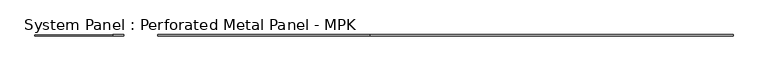
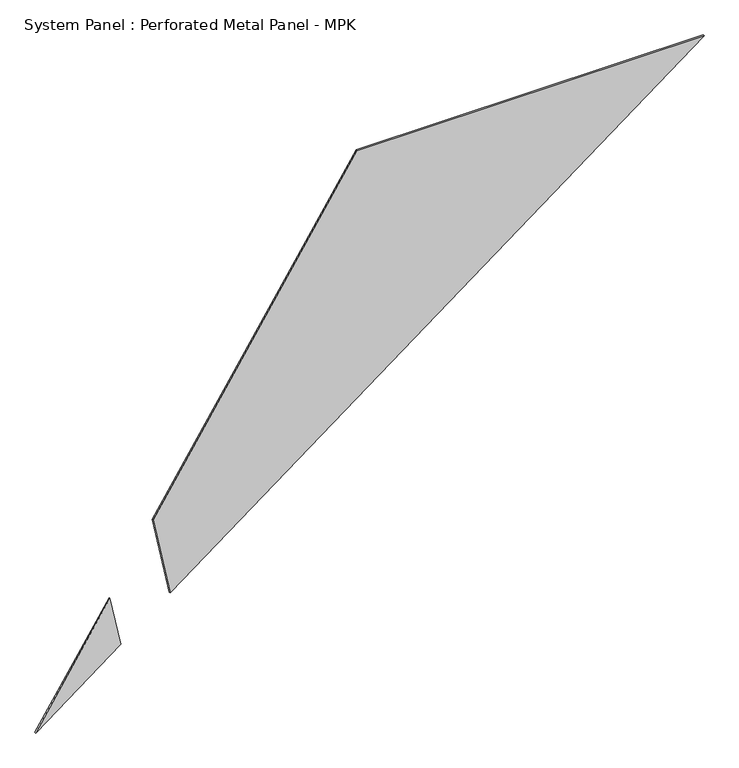
"""IFC4 building model written with IfcOpenShell, lengths in millimetres: plate geometry, System Panel : Perforated Metal Panel - MPK."""

from ifc_helpers import new_model, si_unit, frame, origin, place, context, project, spatial, polyline, outline, extrude, source, transform, mapped, element, save


def system_panel_perforated_metal_panel_mpk_2892176f(model_context):
    return source(origin(), model_context, "Body", "SweptSolid", [
        extrude(outline(polyline([(0.0, -5573.1424665), (1068.2161322, -4154.5434088), (1942.6986226, -4333.5674328), (0.0, -5573.1424665)])), frame((0.0, 0.0, 0.0), z_axis=(0.0, 1.0, 0.0), x_axis=(0.0, 0.0, 1.0)), (0.0, 0.0, 1.0), 20.0),
        extrude(outline(polyline([(3070.7412462, -3613.7988301), (1688.483895, -3330.8231549), (8393.2393128, 5573.1424665), (8393.2393128, -217.6798216), (3070.7412462, -3613.7988301)])), frame((0.0, 0.0, 0.0), z_axis=(0.0, 1.0, 0.0), x_axis=(0.0, 0.0, 1.0)), (0.0, 0.0, 1.0), 20.0),
    ])


if __name__ == "__main__":
    model = new_model("IFC4")
    model_context = context("Model", 3, world=origin())
    ifc_project = project(units=[si_unit("LENGTHUNIT", "METRE", prefix="MILLI")], contexts=[model_context])
    site = spatial("IfcSite", under=ifc_project)
    building = spatial("IfcBuilding", under=site)
    placement = place(None, origin())
    system_panel_perforated_metal_panel_mpk_shape = system_panel_perforated_metal_panel_mpk_2892176f(model_context)
    element("IfcPlate", 1, ObjectType="System Panel : Perforated Metal Panel - MPK", at=placement, inside=building, context=model_context, shape_type="MappedRepresentation", body=[
        mapped(system_panel_perforated_metal_panel_mpk_shape, transform((0.0, 0.0, 0.0), x_axis=(1.0, 0.0, 0.0), y_axis=(0.0, 1.0, 0.0), z_axis=(0.0, 0.0, 1.0))),
    ])
    save(model, "model.ifc")

# Revit data of these elements
# Element 1 (IfcPlate, "System Panel : Perforated Metal Panel - MPK")
#   Materials on its faces: "Perforated  Metal Panels - MPK"
# Materials
#   "Perforated  Metal Panels - MPK": class "Miscellaneous", colour RGB 127 127 127, transparency 0
